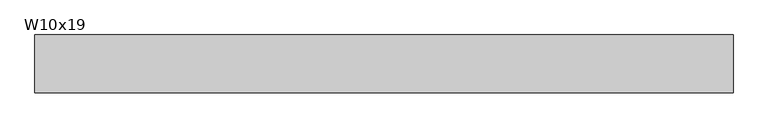
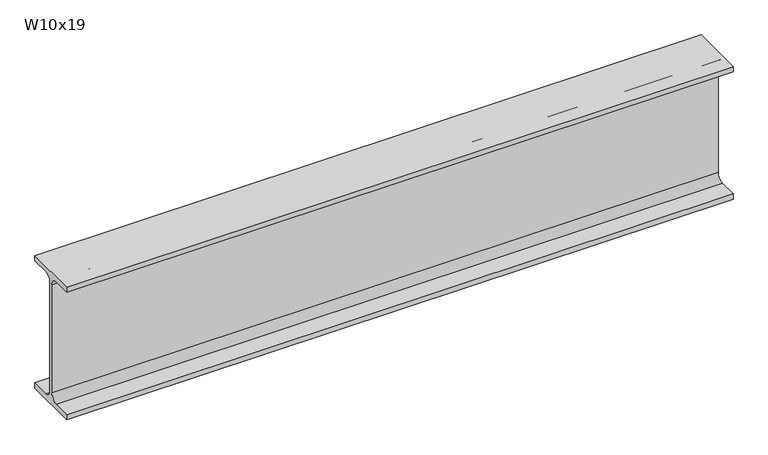
"""IFC4 building model written with IfcOpenShell, lengths in millimetres: beam geometry, RME W-Wide Flange : W10x19."""

from ifc_helpers import new_model, si_unit, point, frame, frame_2d, origin, place, context, project, spatial, polyline, circle_curve, trimmed, segment, composite_curve, outline, extrude, source, transform, mapped, element, save


def w10x19_5b08cad8(model_context):
    return source(origin(), model_context, "Body", "SweptSolid", [
        extrude(outline(composite_curve([segment(polyline([(51.054, -119.507), (51.054, -129.54), (-51.054, -129.54), (-51.054, -119.507), (-16.9545, -119.507)]), True, "CONTINUOUS"), segment(trimmed(circle_curve(frame_2d((-16.9545, -105.7275)), 13.7795), [point((-16.9545, -119.507))], [point((-3.175, -105.7275))], True, "CARTESIAN"), True, "CONTINUOUS"), segment(polyline([(-3.175, -105.7275), (-3.175, 105.7275)]), True, "CONTINUOUS"), segment(trimmed(circle_curve(frame_2d((-16.9545, 105.7275)), 13.7795), [point((-3.175, 105.7275))], [point((-16.9545, 119.507))], True, "CARTESIAN"), True, "CONTINUOUS"), segment(polyline([(-16.9545, 119.507), (-51.054, 119.507), (-51.054, 129.54), (51.054, 129.54), (51.054, 119.507), (16.9545, 119.507)]), True, "CONTINUOUS"), segment(trimmed(circle_curve(frame_2d((16.9545, 105.7275)), 13.7795), [point((16.9545, 119.507))], [point((3.175, 105.7275))], True, "CARTESIAN"), True, "CONTINUOUS"), segment(polyline([(3.175, 105.7275), (3.175, -105.7275)]), True, "CONTINUOUS"), segment(trimmed(circle_curve(frame_2d((16.9545, -105.7275)), 13.7795), [point((3.175, -105.7275))], [point((16.9545, -119.507))], True, "CARTESIAN"), True, "CONTINUOUS"), segment(polyline([(16.9545, -119.507), (51.054, -119.507)]), True, "CONTINUOUS")], self_intersect=False)), frame((-571.5, 0.0, 0.0), z_axis=(1.0, 0.0, 0.0), x_axis=(0.0, 1.0, 0.0)), (0.0, 0.0, 1.0), 1231.9),
    ])


if __name__ == "__main__":
    model = new_model("IFC4")
    model_context = context("Model", 3, world=origin())
    ifc_project = project(units=[si_unit("LENGTHUNIT", "METRE", prefix="MILLI")], contexts=[model_context])
    site = spatial("IfcSite", under=ifc_project)
    building = spatial("IfcBuilding", under=site)
    placement = place(None, origin())
    w10x19_shape = w10x19_5b08cad8(model_context)
    element("IfcBeam", 1, ObjectType="RME W-Wide Flange : W10x19", at=placement, inside=building, context=model_context, shape_type="MappedRepresentation", body=[
        mapped(w10x19_shape, transform((0.0, 0.0, 0.0), x_axis=(1.0, 0.0, 0.0), y_axis=(0.0, 1.0, 0.0), z_axis=(0.0, 0.0, 1.0))),
    ])
    save(model, "model.ifc")

# Revit data of these elements
# Type "RME W-Wide Flange : W10x19"
#   WELD P [instance default] = ""
#   WELD LE [instance default] = ""
#   WELD D [instance default] = ""
#   TOP SECTION SIZE [instance default] = ""
#   TOP SECTION LENGTH [instance default] = ""
#   REMARKS [instance default] = ""
#   REINF TYPE [instance default] = ""
#   Nominal Size = "W24"
#   End Bearing Capacity [instance default] = ""
#   BOT SECTION SIZE [instance default] = ""
#   BOT SECTION LENGTH [instance default] = ""
#   Assembly Code = "B10"
#   W = 19
#   Start Extension Calculation [instance default] = 10' - 0"
#   Start Extension [instance default] = -0' - 0 1/2"
#   End Extension Calculation [instance default] = 10' - 0"
#   End Extension [instance default] = -0' - 0 1/2"
#   Length [instance default] = 5' - 0"
#   bf = 0' - 4.02"
#   d = 0' - 10.2"
#   k = 0' - 0 15/16"
#   k2 = 0' - 0.5425"
#   tf = 0' - 0.395"
#   tw = 0' - 0 1/4"
#   A = 0.0390278 SF
#   Structural Material [instance default] = Metal - Steel - ASTM A992
# Element 1 (IfcBeam, "RME W-Wide Flange : W10x19")
#   Length = 4' - 4"
#   Materials on its faces: "Metal - Steel - ASTM A992"
# Materials
#   "Metal - Steel - ASTM A992": class "Metal", colour RGB 255 128 0, transparency 0
